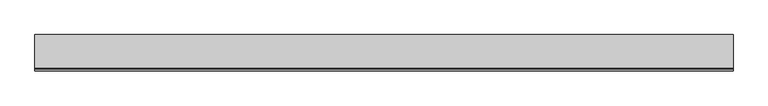
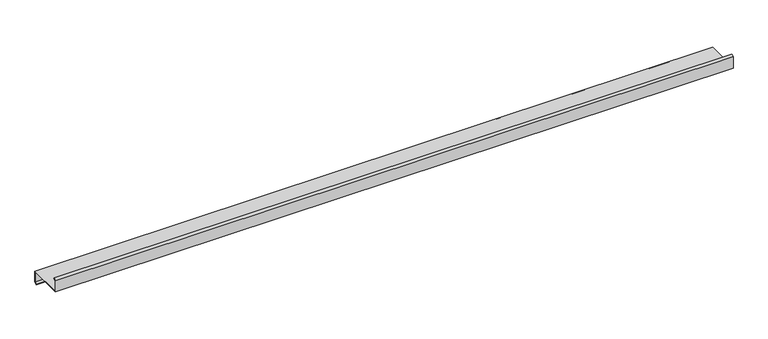
"""IFC4 building model written with IfcOpenShell, lengths in millimetres: proxy geometry, Generic Models 7:Generic Models 1:337419:Generic Models 1:337419 : Generic Models 7:Generic Models 1:337419:20 : Generic Models 7:Generic Models 1:337419:Generic Models 1:337419 : Generic Models 7:Generic Models 1:337419:301336."""

from ifc_helpers import new_model, si_unit, frame, origin, place, context, project, spatial, polyline, outline, extrude, source, transform, mapped, element, save


def generic_models_62c65ba3(model_context):
    return source(origin(), model_context, "Body", "SweptSolid", [
        extrude(outline(polyline([(-536811.2913358, 6126.1625), (-536811.2913358, 6211.8875405), (-536796.8843797, 6223.9764121), (-536794.9124449, 6222.0044772), (-536808.5132108, 6210.5920795), (-536808.5132108, 6128.940625), (-536557.2913358, 6128.940625), (-536557.2913358, 6049.5656655), (-536571.8844825, 6037.3205615), (-536573.8564173, 6039.2924964), (-536560.0694608, 6050.8611264), (-536560.0694608, 6126.1625), (-536811.2913358, 6126.1625)])), frame((591306.0367242, 0.0, 0.0), z_axis=(1.0, 0.0, 0.0), x_axis=(0.0, 1.0, 0.0)), (0.0, 0.0, 1.0), 4876.8),
    ])


if __name__ == "__main__":
    model = new_model("IFC4")
    model_context = context("Model", 3, world=origin())
    ifc_project = project(units=[si_unit("LENGTHUNIT", "METRE", prefix="MILLI")], contexts=[model_context])
    site = spatial("IfcSite", under=ifc_project)
    building = spatial("IfcBuilding", under=site)
    placement = place(None, origin())
    generic_models_shape = generic_models_62c65ba3(model_context)
    element("IfcBuildingElementProxy", 1, Name="Generic Models 7:Generic Models 1:337419:Generic Models 1:337419 : Generic Models 7:Generic Models 1:337419:20 : Generic Models 7:Generic Models 1:337419:Generic Models 1:337419 : Generic Models 7:Generic Models 1:337419:301336", ObjectType="Generic Models 7:Generic Models 1:337419:Generic Models 1:337419 : Generic Models 7:Generic Models 1:337419:20 : Generic Models 7:Generic Models 1:337419:Generic Models 1:337419 : Generic Models 7:Generic Models 1:337419:301336", at=placement, inside=building, context=model_context, shape_type="MappedRepresentation", body=[
        mapped(generic_models_shape, transform((0.0, 0.0, 0.0), x_axis=(1.0, 0.0, 0.0), y_axis=(0.0, 1.0, 0.0), z_axis=(0.0, 0.0, 1.0))),
    ])
    save(model, "model.ifc")

# Revit data of these elements
# Type "Generic Models 7:Generic Models 1:337419:Generic Models 1:337419 : Generic Models 7:Generic Models 1:337419:20 : Generic Models 7:Generic Models 1:337419:Generic Models 1:337419 : Generic Models 7:Generic Models 1:337419:301336"
#   NameOverride = "Generic Models 7:Generic Models 1:337419:Generic Models 1:337419 : Generic Models 7:Generic Models 1:337419:301336"
#   ObjectTypeOverride = "Generic Models 1:337419 : Generic Models 7:Generic Models 1:337419"
#   Reference = "Generic Models 1"
#   Tag = "301336"
# Element 1 (IfcBuildingElementProxy, "Generic Models 7:Generic Models 1:337419:Generic Models 1:337419 : Generic Models 7:Generic Models 1:337419:20 : Generic Models 7:Generic Models 1:337419:Generic Models 1:337419 : Generic Models 7:Generic Models 1:337419:301336")
#   Materials on its faces: "'ZEE' SECTION (8.0x3.5Z - SEE STRUCT. DWGS)"
# Materials
#   "'ZEE' SECTION (8.0x3.5Z - SEE STRUCT. DWGS)": class "Unassigned", colour RGB 210 209 208, transparency 0, Keynote = "M05121300.02", Cost = 0
